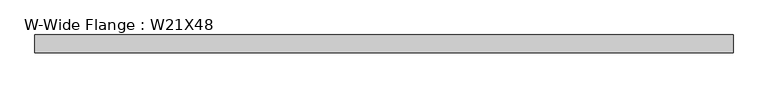
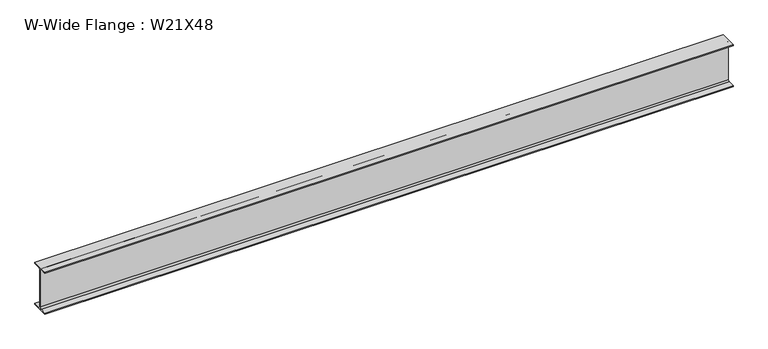
"""IFC4 building model written with IfcOpenShell, lengths in millimetres: beam geometry, W-Wide Flange : W21X48."""

from ifc_helpers import new_model, si_unit, point, frame, frame_2d, origin, place, context, project, spatial, polyline, circle_curve, trimmed, segment, composite_curve, outline, extrude, source, transform, mapped, element, save


def w_wide_flange_w21x48_f7f014d3(model_context):
    return source(origin(), model_context, "Body", "SweptSolid", [
        extrude(outline(composite_curve([segment(polyline([(103.378, -250.698), (103.378, -261.62), (-103.378, -261.62), (-103.378, -250.698), (-22.098, -250.698)]), True, "CONTINUOUS"), segment(trimmed(circle_curve(frame_2d((-22.098, -233.045)), 17.653), [point((-22.098, -250.698))], [point((-4.445, -233.045))], True, "CARTESIAN"), True, "CONTINUOUS"), segment(polyline([(-4.445, -233.045), (-4.445, 233.045)]), True, "CONTINUOUS"), segment(trimmed(circle_curve(frame_2d((-22.098, 233.045)), 17.653), [point((-4.445, 233.045))], [point((-22.098, 250.698))], True, "CARTESIAN"), True, "CONTINUOUS"), segment(polyline([(-22.098, 250.698), (-103.378, 250.698), (-103.378, 261.62), (103.378, 261.62), (103.378, 250.698), (22.098, 250.698)]), True, "CONTINUOUS"), segment(trimmed(circle_curve(frame_2d((22.098, 233.045)), 17.653), [point((22.098, 250.698))], [point((4.445, 233.045))], True, "CARTESIAN"), True, "CONTINUOUS"), segment(polyline([(4.445, 233.045), (4.445, -233.045)]), True, "CONTINUOUS"), segment(trimmed(circle_curve(frame_2d((22.098, -233.045)), 17.653), [point((4.445, -233.045))], [point((22.098, -250.698))], True, "CARTESIAN"), True, "CONTINUOUS"), segment(polyline([(22.098, -250.698), (103.378, -250.698)]), True, "CONTINUOUS")], self_intersect=False)), frame((-4076.7, 0.0, 0.0), z_axis=(1.0, 0.0, 0.0), x_axis=(0.0, 1.0, 0.0)), (0.0, 0.0, 1.0), 8153.4),
    ])


if __name__ == "__main__":
    model = new_model("IFC4")
    model_context = context("Model", 3, world=origin())
    ifc_project = project(units=[si_unit("LENGTHUNIT", "METRE", prefix="MILLI")], contexts=[model_context])
    site = spatial("IfcSite", under=ifc_project)
    building = spatial("IfcBuilding", under=site)
    placement = place(None, origin())
    w_wide_flange_w21x48_shape = w_wide_flange_w21x48_f7f014d3(model_context)
    element("IfcBeam", 1, ObjectType="W-Wide Flange : W21X48", at=placement, inside=building, context=model_context, shape_type="MappedRepresentation", body=[
        mapped(w_wide_flange_w21x48_shape, transform((0.0, 0.0, 0.0), x_axis=(1.0, 0.0, 0.0), y_axis=(0.0, 1.0, 0.0), z_axis=(0.0, 0.0, 1.0))),
    ])
    save(model, "model.ifc")

# Revit data of these elements
# Type "W-Wide Flange : W21X48"
#   Assembly Code = "B10"
#   W = 48
#   Length [instance default] = 5' - 0"
#   bf = 0' - 8.14"
#   d = 1' - 8.6"
#   k = 0' - 1 1/8"
#   k2 = 0' - 0.695"
#   tf = 0' - 0.43"
#   tw = 0' - 0.35"
#   A = 0.0979167 SF
#   Structural Material [instance default] = Steel ASTM A992
# Element 1 (IfcBeam, "W-Wide Flange : W21X48")
#   Materials on its faces: "Steel ASTM A992"
# Materials
#   "Steel ASTM A992": class "Metal", colour RGB 199 199 199, transparency 0, Description = "Structural steel 50ksi", Cost = 0
